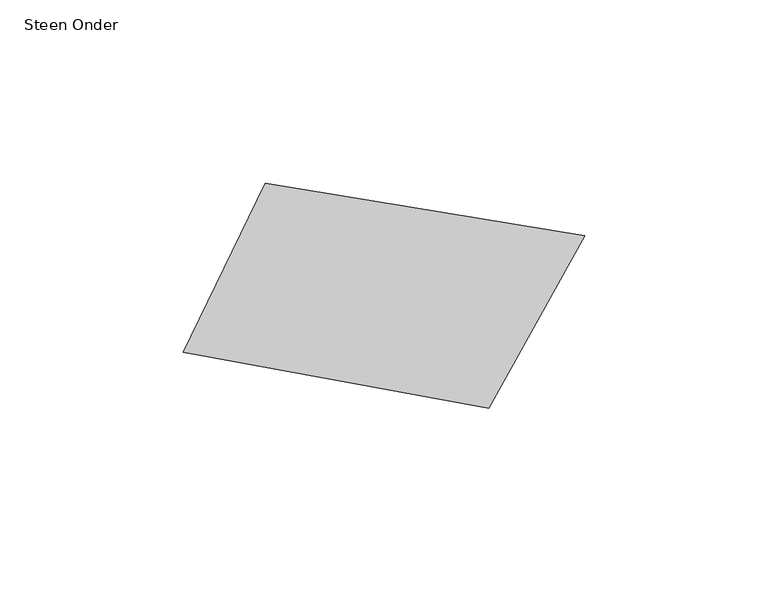
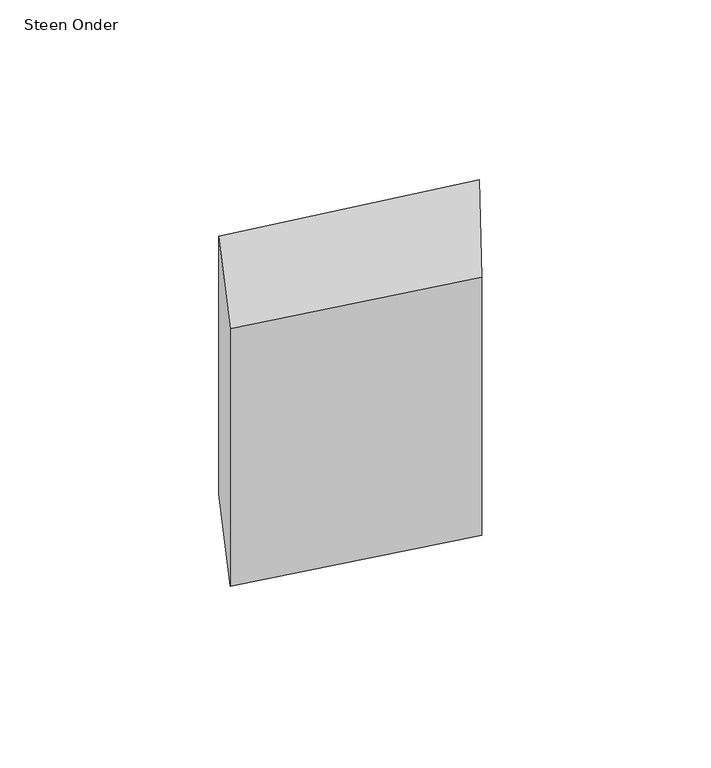
"""IFC4 building model written with IfcOpenShell, lengths in millimetres: proxy geometry, 00_GMA_steen_versie_4 : Steen Onder."""

from ifc_helpers import new_model, si_unit, frame, origin, place, context, project, spatial, polyline, outline, extrude, source, transform, mapped, element, save


def steen_onder_6bde1011(model_context):
    return source(origin(), model_context, "Body", "SweptSolid", [
        extrude(outline(polyline([(144.4321565, 57.3466277), (118.1965574, 10.2395635), (34.7405152, 25.6483654), (57.2094936, 71.7589009), (144.4321565, 57.3466277)])), frame((0.0, 0.0, -100.0), z_axis=(0.0, 0.0, 1.0), x_axis=(1.0, 0.0, 0.0)), (0.0, 0.0, 1.0), 100.0),
    ])


if __name__ == "__main__":
    model = new_model("IFC4")
    model_context = context("Model", 3, world=origin())
    ifc_project = project(units=[si_unit("LENGTHUNIT", "METRE", prefix="MILLI")], contexts=[model_context])
    site = spatial("IfcSite", under=ifc_project)
    building = spatial("IfcBuilding", under=site)
    placement = place(None, origin())
    steen_onder_shape = steen_onder_6bde1011(model_context)
    element("IfcBuildingElementProxy", 1, Name="00_GMA_steen_versie_4 : Steen Onder", ObjectType="00_GMA_steen_versie_4 : Steen Onder", at=placement, inside=building, context=model_context, shape_type="MappedRepresentation", body=[
        mapped(steen_onder_shape, transform((0.0, 0.0, 0.0), x_axis=(1.0, 0.0, 0.0), y_axis=(0.0, 1.0, 0.0), z_axis=(0.0, 0.0, 1.0))),
    ])
    save(model, "model.ifc")

# Revit data of these elements
# Type "00_GMA_steen_versie_4 : Steen Onder"
#   StootVoegHalfBoven [instance default] = 5 mm
#   StootVoegHalf [instance default] = 5 mm
#   StootVoegBreedteOnder = 10 mm
#   StootVoegBreedteBoven = 10 mm
#   Steendikte = 100 mm
#   LintVoegOnderHalf = 0 mm
#   LintVoegOnder = 0 mm
#   LintVoegBovenHalf = 5 mm
#   LintVoegBoven = 10 mm
#   materiaal = none
#   MateriaalVoeg = none
#   Default Elevation = 0
